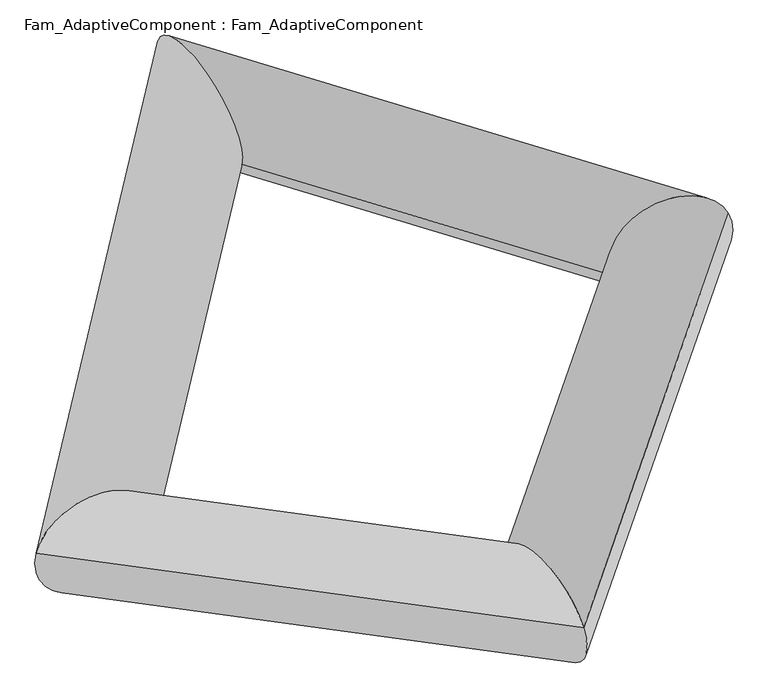
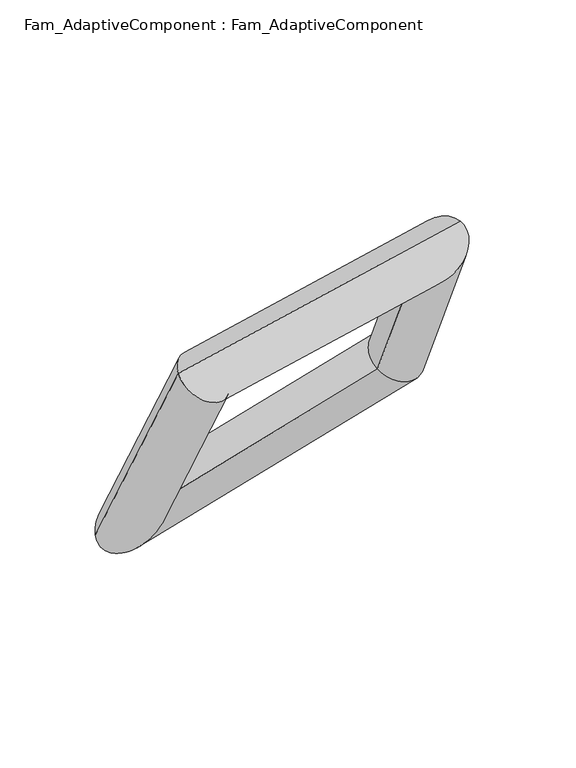
"""IFC4 building model written with IfcOpenShell, lengths in millimetres: proxy geometry, Fam_AdaptiveComponent : Fam_AdaptiveComponent."""

from ifc_helpers import new_model, si_unit, frame, origin, place, context, project, spatial, ellipse_curve, source, transform, mapped, element, save
from ifc_brep_helpers import cylinder_surface, advanced_brep


def fam_adaptivecomponent_fam_adaptivecomponent_f0eaef9a(model_context):
    return source(origin(), model_context, "Body", "AdvancedBrep", [
        advanced_brep(
        [(4397.4108724, 1973.8696358, 10436.4396875), (7939.8054731, 3900.4605356, 9930.6303256), (3475.2652289, -8866.5607114, 27450.5203392), (1141.8382586, -7335.9276687, 23212.0606932), (-13399.5127204, -6574.1175728, 21548.8706586), (-9734.9307402, -5858.3156648, 19408.1066216), (-9651.5442809, 9199.8150985, -372.9793962), (-7054.2737265, 5423.6638745, 3728.9561564)],
        [
            (0, 1, ellipse_curve(frame((6168.6081727, 2937.1650857, 10183.5350065), z_axis=(0.38352033640668287, -0.5015854821231669, 0.775450936994582), x_axis=(0.9192221560366236, 0.2883521952759337, -0.268111244320209)), 2058.6339469, 1700.0)),
            (1, 2),
            (2, 3, ellipse_curve(frame((2308.5517437, -8101.2441901, 25331.2905162), z_axis=(0.8695792851036982, 0.34358498112087116, -0.35465649249197706), x_axis=(-0.4856841437649115, 0.4654936574705939, -0.7398828064970792)), 2598.0775189, 1700.0)),
            (3, 0),
            (1, 0, ellipse_curve(frame((6168.6081727, 2937.1650857, 10183.5350065), z_axis=(0.38352033640668287, -0.5015854821231669, 0.775450936994582), x_axis=(0.9192221560366236, 0.2883521952759337, -0.268111244320209)), 2058.6339469, 1700.0)),
            (3, 2, ellipse_curve(frame((2308.5517437, -8101.2441901, 25331.2905162), z_axis=(0.8695792851036982, 0.34358498112087116, -0.35465649249197706), x_axis=(-0.4856841437649115, 0.4654936574705939, -0.7398828064970792)), 2598.0775189, 1700.0)),
            (2, 4),
            (4, 5, ellipse_curve(frame((-11567.2217303, -6216.2166188, 20478.4886401), z_axis=(0.5138882275624189, -0.4539974756297928, 0.7278771748684878), x_axis=(0.8532151605303726, 0.3586380857061274, -0.37868537510996475)), 2187.2761029, 1700.0)),
            (5, 3),
            (5, 4, ellipse_curve(frame((-11567.2217303, -6216.2166188, 20478.4886401), z_axis=(0.5138882275624189, -0.4539974756297928, 0.7278771748684878), x_axis=(0.8532151605303726, 0.3586380857061274, -0.37868537510996475)), 2187.2761029, 1700.0)),
            (4, 6),
            (6, 7, ellipse_curve(frame((-8352.9090037, 7311.7394865, 1677.9883801), z_axis=(-0.9061756053545301, -0.3046163091555693, 0.2933507737449989), x_axis=(0.4134041519463308, -0.49187792041686373, 0.7662591719254762)), 3167.8354698, 1700.0)),
            (7, 5),
            (7, 6, ellipse_curve(frame((-8352.9090037, 7311.7394865, 1677.9883801), z_axis=(-0.9061756053545301, -0.3046163091555693, 0.2933507737449989), x_axis=(0.4134041519463308, -0.49187792041686373, 0.7662591719254762)), 3167.8354698, 1700.0)),
            (6, 1),
            (0, 7),
        ],
        [
            cylinder_surface(frame((6168.6081727, 2937.1650857, 10183.5350065), z_axis=(0.2017129976597878, 0.5768285167305944, -0.7915685244257034), x_axis=(0.4998058712762529, 0.6344142105054544, 0.5896716887781938)), 1700.0),
            cylinder_surface(frame((2308.5517437, -8101.2441901, 25331.2905162), z_axis=(0.936270587447429, -0.12719261198580994, 0.32744377614649167), x_axis=(-0.2714503169523101, 0.329678291180668, 0.9042272666485375)), 1700.0),
            cylinder_surface(frame((-11567.2217303, -6216.2166188, 20478.4886401), z_axis=(-0.13745969593253377, -0.5785214106404366, 0.8040011252633511), x_axis=(-0.6506979316913666, 0.6647267521015565, 0.3670565988142611)), 1700.0),
            cylinder_surface(frame((-8352.9090037, 7311.7394865, 1677.9883801), z_axis=(-0.835127765614034, 0.25158036177895315, -0.4891512410979675), x_axis=(0.24611927124139182, 0.966197178727881, 0.07673536434975263)), 1700.0),
        ],
        [
            (0, [[1, 2, 3, 4]]),
            (0, [[5, -4, 6, -2]]),
            (1, [[-3, 7, 8, 9]]),
            (1, [[-6, -9, 10, -7]]),
            (2, [[-8, 11, 12, 13]]),
            (2, [[-10, -13, 14, -11]]),
            (3, [[-12, 15, -1, 16]]),
            (3, [[-14, -16, -5, -15]]),
        ],
    ),
    ])


if __name__ == "__main__":
    model = new_model("IFC4")
    model_context = context("Model", 3, world=origin())
    ifc_project = project(units=[si_unit("LENGTHUNIT", "METRE", prefix="MILLI")], contexts=[model_context])
    site = spatial("IfcSite", under=ifc_project)
    building = spatial("IfcBuilding", under=site)
    placement = place(None, origin())
    fam_adaptivecomponent_fam_adaptivecomponent_shape = fam_adaptivecomponent_fam_adaptivecomponent_f0eaef9a(model_context)
    element("IfcBuildingElementProxy", 1, Name="Fam_AdaptiveComponent : Fam_AdaptiveComponent", ObjectType="Fam_AdaptiveComponent : Fam_AdaptiveComponent", at=placement, inside=building, context=model_context, shape_type="MappedRepresentation", body=[
        mapped(fam_adaptivecomponent_fam_adaptivecomponent_shape, transform((0.0, 0.0, 0.0), x_axis=(1.0, 0.0, 0.0), y_axis=(0.0, 1.0, 0.0), z_axis=(0.0, 0.0, 1.0))),
    ])
    save(model, "model.ifc")

# Revit data of these elements
# Type "Fam_AdaptiveComponent : Fam_AdaptiveComponent"
#   Default Elevation = 0
